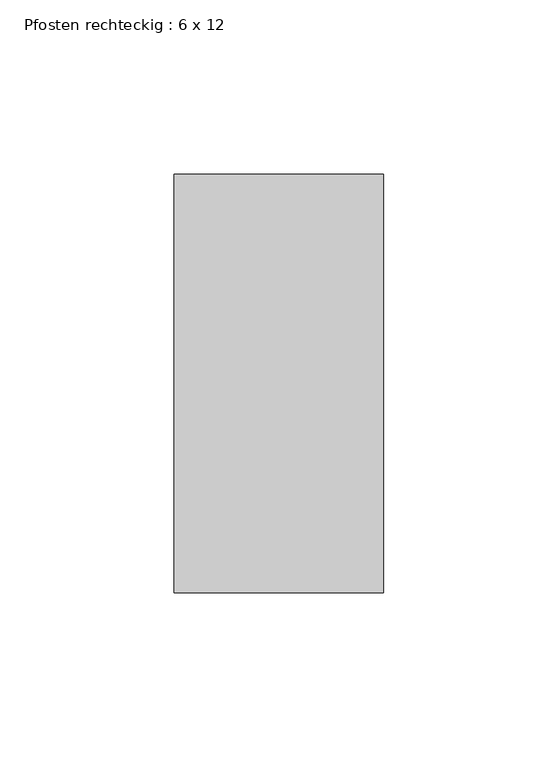
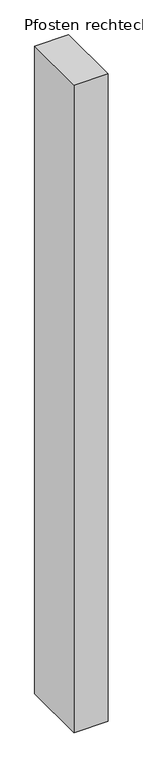
"""IFC4 building model written with IfcOpenShell, lengths in millimetres: member geometry, Pfosten rechteckig : 6 x 12."""

from ifc_helpers import new_model, si_unit, frame, origin, place, context, project, spatial, polyline, outline, extrude, source, transform, mapped, element, save


def pfosten_rechteckig_6_x_12_9195eeaf(model_context):
    return source(origin(), model_context, "Body", "SweptSolid", [
        extrude(outline(polyline([(0.0, 60.0), (0.0, -60.0), (-60.0, -60.0), (-60.0, 60.0), (0.0, 60.0)])), frame((0.0, 0.0, -1210.0000003), z_axis=(0.0, 0.0, 1.0), x_axis=(1.0, 0.0, 0.0)), (0.0, 0.0, 1.0), 1210.0000003),
    ])


if __name__ == "__main__":
    model = new_model("IFC4")
    model_context = context("Model", 3, world=origin())
    ifc_project = project(units=[si_unit("LENGTHUNIT", "METRE", prefix="MILLI")], contexts=[model_context])
    site = spatial("IfcSite", under=ifc_project)
    building = spatial("IfcBuilding", under=site)
    placement = place(None, origin())
    pfosten_rechteckig_6_x_12_shape = pfosten_rechteckig_6_x_12_9195eeaf(model_context)
    element("IfcMember", 1, ObjectType="Pfosten rechteckig : 6 x 12", at=placement, inside=building, context=model_context, shape_type="MappedRepresentation", body=[
        mapped(pfosten_rechteckig_6_x_12_shape, transform((0.0, 0.0, 0.0), x_axis=(1.0, 0.0, 0.0), y_axis=(0.0, 1.0, 0.0), z_axis=(0.0, 0.0, 1.0))),
    ])
    save(model, "model.ifc")

# Revit data of these elements
# Type "Pfosten rechteckig : 6 x 12"
#   built-in parameter 1007304 = 0.393701 (stored number, unit not read)
#   built-in parameter 1007301 = 0.0984252 (stored number, unit not read)
#   built-in parameter 1007300 = 0.0984252 (stored number, unit not read)
# Element 1 (IfcMember, "Pfosten rechteckig : 6 x 12")
#   Materials on its faces: "Metall - verzinkt"
# Materials
#   "Metall - verzinkt": class "Allgemeines", colour RGB 200 200 200, transparency 0, Cost = 0
